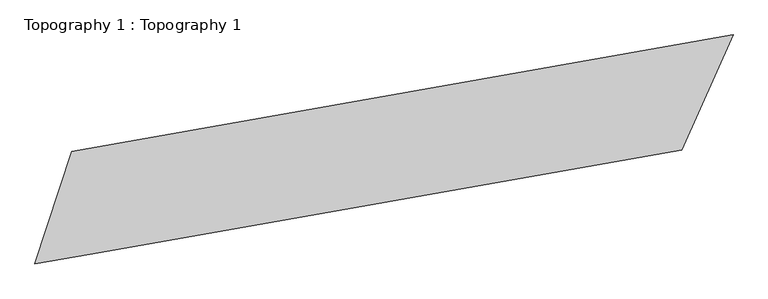
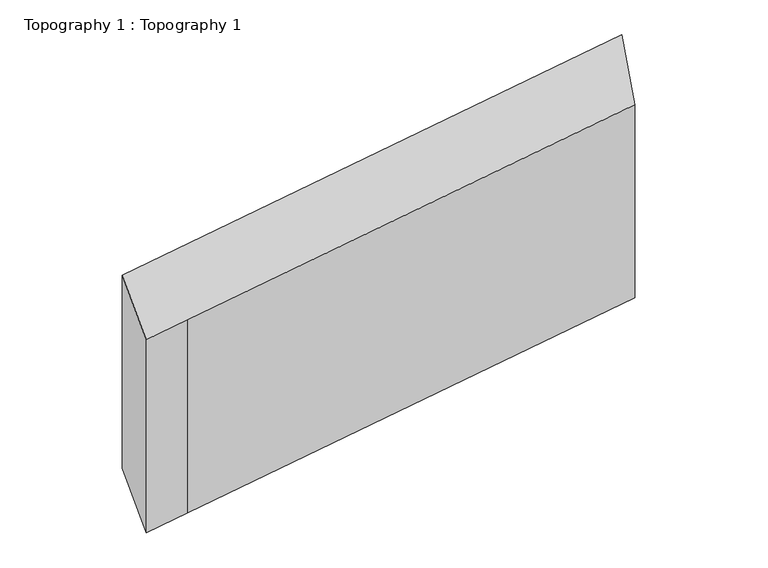
"""IFC4 building model written with IfcOpenShell, lengths in millimetres: proxy geometry, Topography 1 : Topography 1."""

from ifc_helpers import new_model, si_unit, frame, origin, place, context, project, spatial, polyline, outline, extrude, source, transform, mapped, element, save


def topography_1_topography_1_8be638cc(model_context):
    return source(origin(), model_context, "Body", "SweptSolid", [
        extrude(outline(polyline([(152555.8202257, 96707.6433044), (149937.6623725, 96245.9914351), (151687.5793374, 101631.6820694), (183270.7060146, 107200.6394378), (180817.6408186, 101690.9647988), (152555.8202257, 96707.6433044)])), frame((0.0, 0.0, -10770.0), z_axis=(0.0, 0.0, 1.0), x_axis=(1.0, 0.0, 0.0)), (0.0, 0.0, 1.0), 11590.6948414),
    ])


if __name__ == "__main__":
    model = new_model("IFC4")
    model_context = context("Model", 3, world=origin())
    ifc_project = project(units=[si_unit("LENGTHUNIT", "METRE", prefix="MILLI")], contexts=[model_context])
    site = spatial("IfcSite", under=ifc_project)
    building = spatial("IfcBuilding", under=site)
    placement = place(None, origin())
    topography_1_topography_1_shape = topography_1_topography_1_8be638cc(model_context)
    element("IfcBuildingElementProxy", 1, Name="Topography 1 : Topography 1", ObjectType="Topography 1 : Topography 1", at=placement, inside=building, context=model_context, shape_type="MappedRepresentation", body=[
        mapped(topography_1_topography_1_shape, transform((0.0, 0.0, 0.0), x_axis=(1.0, 0.0, 0.0), y_axis=(0.0, 1.0, 0.0), z_axis=(0.0, 0.0, 1.0))),
    ])
    save(model, "model.ifc")

# Revit data of these elements
# Element 1 (IfcBuildingElementProxy, "Topography 1 : Topography 1")
#   Materials on its faces: "Earth"
# Materials
#   "Earth": class "Generic", colour RGB 97 75 62, transparency 0, Description = "Soil", Cost = 0
